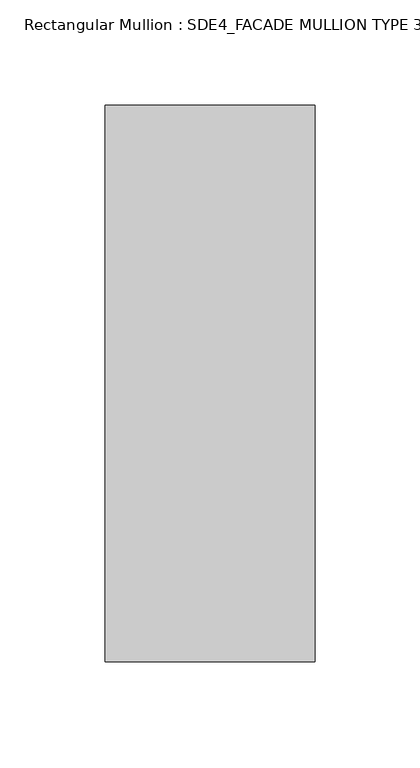
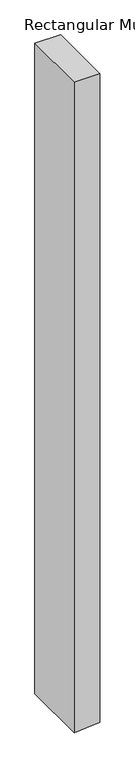
"""IFC4 building model written with IfcOpenShell, lengths in millimetres: member geometry, Rectangular Mullion : SDE4_FACADE MULLION TYPE 3."""

from ifc_helpers import new_model, si_unit, frame, origin, place, context, project, spatial, polyline, outline, extrude, source, transform, mapped, element, save


def rectangular_mullion_sde4_facade_mullion_type_3_763ea594(model_context):
    return source(origin(), model_context, "Body", "SweptSolid", [
        extrude(outline(polyline([(0.0, 50.0), (0.0, -50.0), (-2678.2810458, -50.0), (-2674.6834485, -3.056508), (-2670.6173694, 50.0), (0.0, 50.0)])), frame((0.0, -132.5, 0.0), z_axis=(0.0, 1.0, 0.0), x_axis=(0.0, 0.0, 1.0)), (0.0, 0.0, 1.0), 265.0),
    ])


if __name__ == "__main__":
    model = new_model("IFC4")
    model_context = context("Model", 3, world=origin())
    ifc_project = project(units=[si_unit("LENGTHUNIT", "METRE", prefix="MILLI")], contexts=[model_context])
    site = spatial("IfcSite", under=ifc_project)
    building = spatial("IfcBuilding", under=site)
    placement = place(None, origin())
    rectangular_mullion_sde4_facade_mullion_type_3_shape = rectangular_mullion_sde4_facade_mullion_type_3_763ea594(model_context)
    element("IfcMember", 1, ObjectType="Rectangular Mullion : SDE4_FACADE MULLION TYPE 3", at=placement, inside=building, context=model_context, shape_type="MappedRepresentation", body=[
        mapped(rectangular_mullion_sde4_facade_mullion_type_3_shape, transform((0.0, 0.0, 0.0), x_axis=(1.0, 0.0, 0.0), y_axis=(0.0, 1.0, 0.0), z_axis=(0.0, 0.0, 1.0))),
    ])
    save(model, "model.ifc")

# Revit data of these elements
# Type "Rectangular Mullion : SDE4_FACADE MULLION TYPE 3"
#   built-in parameter 1007322 = 0.869423 (stored number, unit not read)
#   built-in parameter 1007321 = 0.164042 (stored number, unit not read)
#   built-in parameter 1007320 = 0.164042 (stored number, unit not read)
